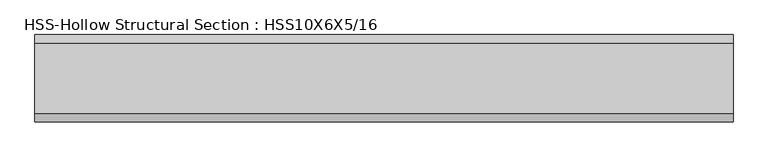
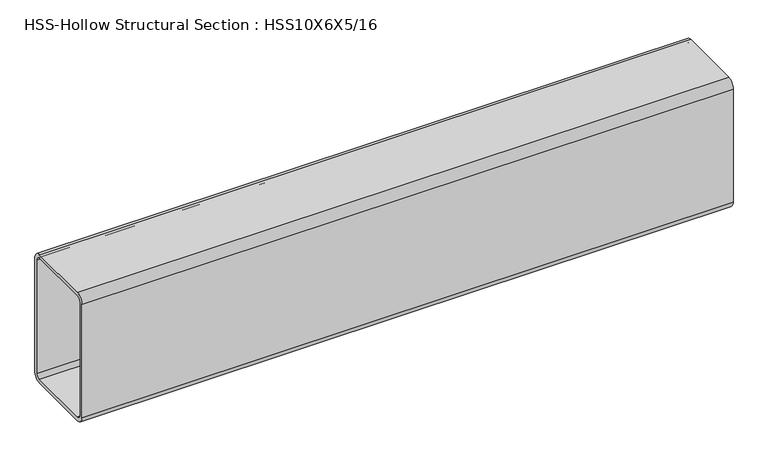
"""IFC4 building model written with IfcOpenShell, lengths in millimetres: beam geometry, HSS-Hollow Structural Section : HSS10X6X5/16."""

from ifc_helpers import new_model, si_unit, point, frame, frame_2d, origin, place, context, project, spatial, polyline, circle_curve, trimmed, segment, composite_curve, outline, extrude, source, transform, mapped, element, save


def hss_hollow_structural_section_hss10x6x5_16_9f903aa6(model_context):
    return source(origin(), model_context, "Body", "SweptSolid", [
        extrude(outline(composite_curve([segment(polyline([(76.2, 112.2172), (76.2, -112.2172)]), True, "CONTINUOUS"), segment(trimmed(circle_curve(frame_2d((61.4172, -112.2172)), 14.7828), [point((76.2, -112.2172))], [point((61.4172, -127.0))], False, "CARTESIAN"), True, "CONTINUOUS"), segment(polyline([(61.4172, -127.0), (-61.4172, -127.0)]), True, "CONTINUOUS"), segment(trimmed(circle_curve(frame_2d((-61.4172, -112.2172)), 14.7828), [point((-61.4172, -127.0))], [point((-76.2, -112.2172))], False, "CARTESIAN"), True, "CONTINUOUS"), segment(polyline([(-76.2, -112.2172), (-76.2, 112.2172)]), True, "CONTINUOUS"), segment(trimmed(circle_curve(frame_2d((-61.4172, 112.2172)), 14.7828), [point((-76.2, 112.2172))], [point((-61.4172, 127.0))], False, "CARTESIAN"), True, "CONTINUOUS"), segment(polyline([(-61.4172, 127.0), (61.4172, 127.0)]), True, "CONTINUOUS"), segment(trimmed(circle_curve(frame_2d((61.4172, 112.2172)), 14.7828), [point((61.4172, 127.0))], [point((76.2, 112.2172))], False, "CARTESIAN"), True, "CONTINUOUS")], self_intersect=False), holes=[composite_curve([segment(trimmed(circle_curve(frame_2d((-61.4172, 112.2172)), 7.3914), [point((-61.4172, 119.6086))], [point((-68.8086, 112.2172))], True, "CARTESIAN"), True, "CONTINUOUS"), segment(polyline([(-68.8086, 112.2172), (-68.8086, -112.2172)]), True, "CONTINUOUS"), segment(trimmed(circle_curve(frame_2d((-61.4172, -112.2172)), 7.3914), [point((-68.8086, -112.2172))], [point((-61.4172, -119.6086))], True, "CARTESIAN"), True, "CONTINUOUS"), segment(polyline([(-61.4172, -119.6086), (61.4172, -119.6086)]), True, "CONTINUOUS"), segment(trimmed(circle_curve(frame_2d((61.4172, -112.2172)), 7.3914), [point((61.4172, -119.6086))], [point((68.8086, -112.2172))], True, "CARTESIAN"), True, "CONTINUOUS"), segment(polyline([(68.8086, -112.2172), (68.8086, 112.2172)]), True, "CONTINUOUS"), segment(trimmed(circle_curve(frame_2d((61.4172, 112.2172)), 7.3914), [point((68.8086, 112.2172))], [point((61.4172, 119.6086))], True, "CARTESIAN"), True, "CONTINUOUS"), segment(polyline([(61.4172, 119.6086), (-61.4172, 119.6086)]), True, "CONTINUOUS")], self_intersect=False)]), frame((-609.6, 0.0, 0.0), z_axis=(1.0, 0.0, 0.0), x_axis=(0.0, 1.0, 0.0)), (0.0, 0.0, 1.0), 1219.2),
    ])


if __name__ == "__main__":
    model = new_model("IFC4")
    model_context = context("Model", 3, world=origin())
    ifc_project = project(units=[si_unit("LENGTHUNIT", "METRE", prefix="MILLI")], contexts=[model_context])
    site = spatial("IfcSite", under=ifc_project)
    building = spatial("IfcBuilding", under=site)
    placement = place(None, origin())
    hss_hollow_structural_section_hss10x6x5_16_shape = hss_hollow_structural_section_hss10x6x5_16_9f903aa6(model_context)
    element("IfcBeam", 1, ObjectType="HSS-Hollow Structural Section : HSS10X6X5/16", at=placement, inside=building, context=model_context, shape_type="MappedRepresentation", body=[
        mapped(hss_hollow_structural_section_hss10x6x5_16_shape, transform((0.0, 0.0, 0.0), x_axis=(1.0, 0.0, 0.0), y_axis=(0.0, 1.0, 0.0), z_axis=(0.0, 0.0, 1.0))),
    ])
    save(model, "model.ifc")

# Revit data of these elements
# Type "HSS-Hollow Structural Section : HSS10X6X5/16"
#   Assembly Code = "B10"
#   Shape = "Rect."
#   W = 31.8
#   Ht = 0' - 10"
#   Length [instance default] = 5' - 0"
#   b = 0' - 6"
#   kr = 0' - 0.582"
#   t = 0' - 0.291"
#   A = 0.0608333 SF
#   Structural Material [instance default] = Steel ASTM A500, Grade B, Rectangular and Square
# Element 1 (IfcBeam, "HSS-Hollow Structural Section : HSS10X6X5/16")
#   Structural Material = Steel ASTM A992
#   Materials on its faces: "Steel ASTM A992"
# Materials
#   "Steel ASTM A500, Grade B, Rectangular and Square": class "Metal", colour RGB 199 199 199, transparency 0, Description = "Carbon steel", Cost = 0
#   "Steel ASTM A992": class "Metal", colour RGB 199 199 199, transparency 0, Description = "Structural steel 50ksi", Cost = 0
